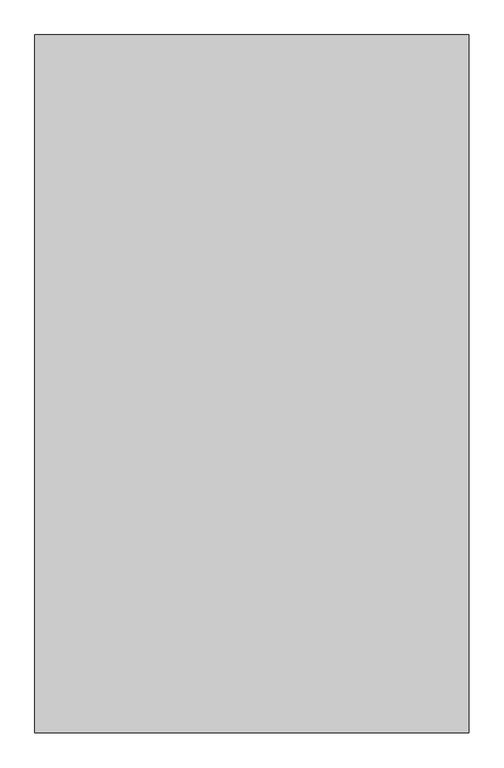
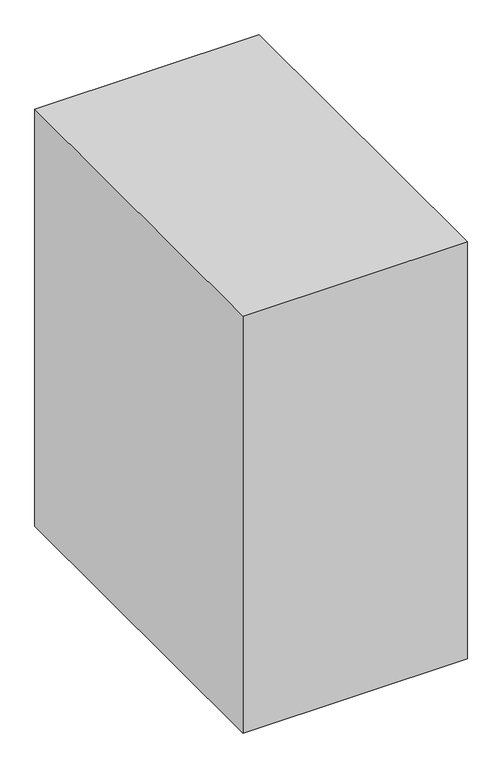
"""IFC4 building model written with IfcOpenShell, lengths in millimetres: proxy geometry, Space Planning Box_hec : Space Planning Box_hec."""

from ifc_helpers import new_model, si_unit, origin, origin_with_axes, place, context, project, spatial, polyline, outline, extrude, source, transform, mapped, element, save


def generic_models_ac48a1a3(model_context):
    return source(origin(), model_context, "Body", "SweptSolid", [
        extrude(outline(polyline([(1400.0, 2250.0), (1400.0, -2250.0), (-1400.0, -2250.0), (-1400.0, 2250.0), (1400.0, 2250.0)])), origin_with_axes(), (0.0, 0.0, 1.0), 5500.0),
    ])


if __name__ == "__main__":
    model = new_model("IFC4")
    model_context = context("Model", 3, world=origin())
    ifc_project = project(units=[si_unit("LENGTHUNIT", "METRE", prefix="MILLI")], contexts=[model_context])
    site = spatial("IfcSite", under=ifc_project)
    building = spatial("IfcBuilding", under=site)
    placement = place(None, origin())
    generic_models_shape = generic_models_ac48a1a3(model_context)
    element("IfcBuildingElementProxy", 1, Name="Space Planning Box_hec : Space Planning Box_hec", ObjectType="Space Planning Box_hec : Space Planning Box_hec", at=placement, inside=building, context=model_context, shape_type="MappedRepresentation", body=[
        mapped(generic_models_shape, transform((0.0, 0.0, 0.0), x_axis=(1.0, 0.0, 0.0), y_axis=(0.0, 1.0, 0.0), z_axis=(0.0, 0.0, 1.0))),
    ])
    save(model, "model.ifc")

# Revit data of these elements
# Type "Space Planning Box_hec : Space Planning Box_hec"
#   Type Comments = "..."
#   Room Name [instance default] = "?"
#   Interior Finish [instance default] = ""
#   Exterior Finish [instance default] = ""
#   Department [instance default] = ""
#   Assembly Code = "..."
#   ceiling height [instance default] = 0
#   Width [instance default] = 1524 mm
#   Program Area [instance default] = 0.00 m²
#   Length [instance default] = 1524 mm
#   Height [instance default] = 1524 mm
#   Area [instance default] = 2.32258 m²
#   Fill Color [instance default] = Cyan
#   Default Elevation = 0
# Element 1 (IfcBuildingElementProxy, "Space Planning Box_hec : Space Planning Box_hec")
#   Room Name = "Toilet"
#   Exterior Finish = "N/A..N/A,,EW2..N/A..N/A"
#   Department = "AR"
#   Width = 2800 mm
#   Program Area = 12.60 m²
#   Length = 4500 mm
#   Height = 5500 mm
#   Area = 12.60 m²
#   Materials on its faces: "Cyan"
# Materials
#   "Cyan": class "Generic", colour RGB 0 255 255, transparency 0.2, Cost = 0
